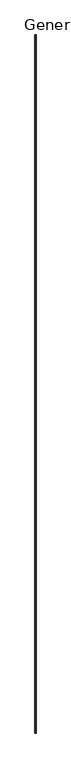
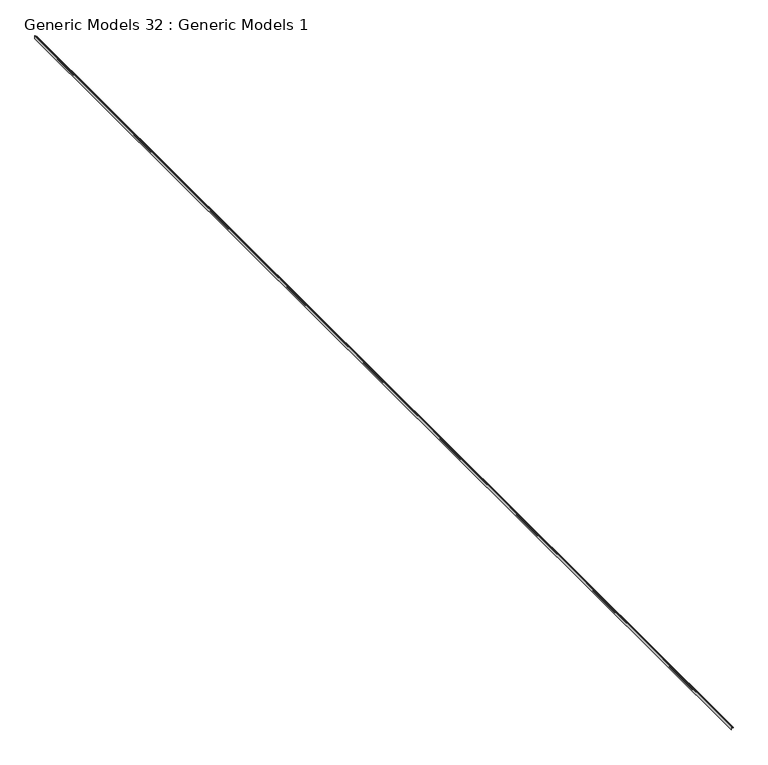
"""IFC4 building model written with IfcOpenShell, lengths in millimetres: proxy geometry, Generic Models 32 : Generic Models 1."""

from ifc_helpers import new_model, si_unit, origin, place, context, project, spatial, faceted_brep, source, transform, mapped, element, save


def generic_models_32_generic_models_1_de8c719f(model_context):
    return source(origin(), model_context, "Body", "Brep", [
        faceted_brep([(-9255.2986296, 7054.2769662, 126669.546), (-9255.2986296, 7054.2769662, 126708.916), (-9254.0286296, 7054.2769662, 126708.916), (-9254.0286296, 7054.2769662, 126689.866), (-9250.8536295, 7054.2769662, 126689.866), (-9234.3436296, 7054.2769662, 126689.866), (-9234.3436296, 7054.2769662, 126693.3458), (-9233.0736296, 7054.2769662, 126693.3458), (-9233.0736296, 7054.2769662, 126688.596), (-9254.0286296, 7054.2769662, 126688.596), (-9254.0286296, 7054.2769662, 126669.546), (-9255.2986296, -7068.1230338, 126669.546), (-9254.0286296, -7068.1230338, 126669.546), (-9254.0286296, -7068.1230338, 126688.596), (-9233.0736296, -7068.1230338, 126688.596), (-9233.0736296, -7068.1230338, 126693.3458), (-9234.3436296, -7068.1230338, 126693.3458), (-9234.3436296, -7068.1230338, 126689.866), (-9254.0286296, -7068.1230338, 126689.866), (-9254.0286296, -7068.1230338, 126708.916), (-9255.2986296, -7068.1230338, 126708.916), (-9233.0736296, -6864.9230338, 126693.3458), (-9234.3436296, -6864.9230338, 126693.3458), (-9234.3436296, -6864.9230338, 126689.866)], [[[0, 1, 2, 3, 4, 5, 6, 7, 8, 9, 10]], [[11, 12, 13, 14, 15, 16, 17, 18, 19, 20]], [[0, 10, 12, 11]], [[10, 9, 13, 12]], [[9, 8, 14, 13]], [[8, 7, 21, 15, 14]], [[7, 6, 22, 16, 15, 21]], [[6, 5, 23, 17, 16, 22]], [[5, 4, 3, 18, 17, 23]], [[3, 2, 19, 18]], [[2, 1, 20, 19]], [[1, 0, 11, 20]]]),
    ])


if __name__ == "__main__":
    model = new_model("IFC4")
    model_context = context("Model", 3, world=origin())
    ifc_project = project(units=[si_unit("LENGTHUNIT", "METRE", prefix="MILLI")], contexts=[model_context])
    site = spatial("IfcSite", under=ifc_project)
    building = spatial("IfcBuilding", under=site)
    placement = place(None, origin())
    generic_models_32_generic_models_1_shape = generic_models_32_generic_models_1_de8c719f(model_context)
    element("IfcBuildingElementProxy", 1, Name="Generic Models 32 : Generic Models 1", ObjectType="Generic Models 32 : Generic Models 1", at=placement, inside=building, context=model_context, shape_type="MappedRepresentation", body=[
        mapped(generic_models_32_generic_models_1_shape, transform((0.0, 0.0, 0.0), x_axis=(1.0, 0.0, 0.0), y_axis=(0.0, 1.0, 0.0), z_axis=(0.0, 0.0, 1.0))),
    ])
    save(model, "model.ifc")

# Revit data of these elements
# Element 1 (IfcBuildingElementProxy, "Generic Models 32 : Generic Models 1")
#   Materials on its faces: "_ 16 GA. COPPER VENTED T REVEAL BEAD (CONT. AROUND PERIMETER OF BEAM)"
# Materials
#   "_ 16 GA. COPPER VENTED T REVEAL BEAD (CONT. AROUND PERIMETER OF BEAM)": class "Generic", colour RGB 253 192 103, transparency 0, Cost = 0
